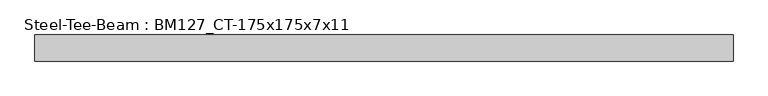
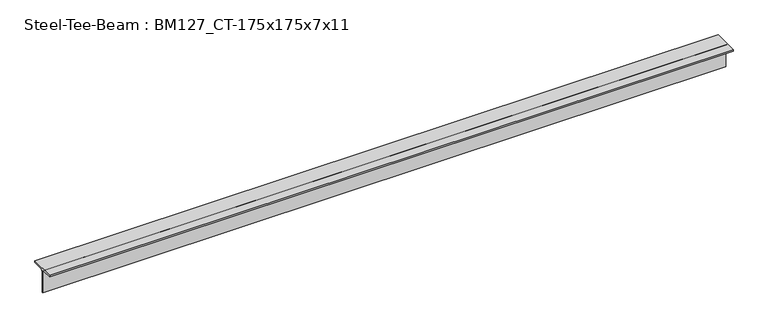
"""IFC4 building model written with IfcOpenShell, lengths in millimetres: beam geometry, Steel-Tee-Beam : BM127_CT-175x175x7x11."""

from ifc_helpers import new_model, si_unit, point, frame, frame_2d, origin, place, context, project, spatial, polyline, circle_curve, trimmed, segment, composite_curve, outline, extrude, source, transform, mapped, element, save


def steel_tee_beam_bm127_ct_175x175x7x11_ea611a39(model_context):
    return source(origin(), model_context, "Body", "SweptSolid", [
        extrude(outline(composite_curve([segment(polyline([(87.5, 87.5), (87.5, 76.5), (17.5, 76.5)]), True, "CONTINUOUS"), segment(trimmed(circle_curve(frame_2d((17.5, 62.5)), 14.0), [point((17.5, 76.5))], [point((3.5, 62.5))], True, "CARTESIAN"), True, "CONTINUOUS"), segment(polyline([(3.5, 62.5), (3.5, -87.5), (-3.5, -87.5), (-3.5, 62.5)]), True, "CONTINUOUS"), segment(trimmed(circle_curve(frame_2d((-17.5, 62.5)), 14.0), [point((-3.5, 62.5))], [point((-17.5, 76.5))], True, "CARTESIAN"), True, "CONTINUOUS"), segment(polyline([(-17.5, 76.5), (-87.5, 76.5), (-87.5, 87.5), (87.5, 87.5)]), True, "CONTINUOUS")], self_intersect=False)), frame((-2302.448777, 0.0, 0.0), z_axis=(1.0, 0.0, 0.0), x_axis=(0.0, 1.0, 0.0)), (0.0, 0.0, 1.0), 4667.7067484),
    ])


if __name__ == "__main__":
    model = new_model("IFC4")
    model_context = context("Model", 3, world=origin())
    ifc_project = project(units=[si_unit("LENGTHUNIT", "METRE", prefix="MILLI")], contexts=[model_context])
    site = spatial("IfcSite", under=ifc_project)
    building = spatial("IfcBuilding", under=site)
    placement = place(None, origin())
    steel_tee_beam_bm127_ct_175x175x7x11_shape = steel_tee_beam_bm127_ct_175x175x7x11_ea611a39(model_context)
    element("IfcBeam", 1, ObjectType="Steel-Tee-Beam : BM127_CT-175x175x7x11", at=placement, inside=building, context=model_context, shape_type="MappedRepresentation", body=[
        mapped(steel_tee_beam_bm127_ct_175x175x7x11_shape, transform((0.0, 0.0, 0.0), x_axis=(1.0, 0.0, 0.0), y_axis=(0.0, 1.0, 0.0), z_axis=(0.0, 0.0, 1.0))),
    ])
    save(model, "model.ifc")

# Revit data of these elements
# Type "Steel-Tee-Beam : BM127_CT-175x175x7x11"
#   Surface Area = 0.00 m²/m
#   Section Area = 31.57 cm²
#   Mass per Unit Length = 24.80 kg/m
#   Length [instance default] = 1524 mm
#   bf = 175 mm
#   d = 175 mm
#   k = 25 mm
#   kr = 14 mm
#   tf = 11 mm
#   tw = 7 mm
#   hec_material4 [instance default] = none
#   hec_material3 [instance default] = none
#   hec_material2 [instance default] = none
#   hec_material1 [instance default] = none
#   Structural Material [instance default] = Steel, 45-345
#   Assembly Code = ""
# Element 1 (IfcBeam, "Steel-Tee-Beam : BM127_CT-175x175x7x11")
#   hec_material3 = F01AC000-00002_Building/Shelter Fire Proofing Work_Intumescent Coating Type_1 hr. rating (UL 1709))
#   hec_material2 = S01AA010-00002_Main Steel Structure Fabrication Work_Shelter/Building_Steel Painting/Coating_for Fireproofed Steel Surface, Surface Preparation & Primer Coat
#   hec_material1 = S03AA029-00001_Main Steel Structure Erection Work_Shelter/Building_Light Steel
#   Structural Material = S01AA003-00001_Main Steel Structure Fabrication Work_Shelter/Building_Light Steel - Standard
#   Materials on its faces: "S01AA003-00001_Main Steel Structure Fabrication Work_Shelter/Building_Light Steel - Standard"
# Materials
#   "Steel, 45-345": class "Metal", colour RGB 189 187 185, transparency 0, Description = "Steel 345 MPa", Cost = 0
#   "S01AA003-00001_Main Steel Structure Fabrication Work_Shelter/Building_Light Steel - Standard": class "Metal", colour RGB 120 120 120, transparency 0, Comments = "(30KG/M>Weight)", Description = "Structural steel 50ksi", W00) Work Master Code = "S01AA003-00001", W01) Work Master_Lv1 = "Main Steel Structure Fabrication Work", W02) Work Master_Lv2 = "Shelter/Building", W03) Work Master_Spec.1 = "Light Steel - Standard (30KG/M>Weight)", Cost = 0
#   "F01AC000-00002_Building/Shelter Fire Proofing Work_Intumescent Coating Type_1 hr. rating (UL 1709))": class "Metal", colour RGB 255 128 128, transparency 0, Description = "Paint finished steel", W00) Work Master Code = "F01AC000-00002", W01) Work Master_Lv1 = "Building/Shelter Fire Proofing Work", W02) Work Master_Lv2 = "Intumescent Coating Type", W03) Work Master_Spec.1 = "1 hr. rating (UL 1709)", Cost = 0
#   "S01AA010-00002_Main Steel Structure Fabrication Work_Shelter/Building_Steel Painting/Coating_for Fireproofed Steel Surface, Surface Preparation & Primer Coat": class "Metal", colour RGB 120 120 120, transparency 0, Description = "Paint finished steel", W00) Work Master Code = "SS01AA010-00002", W01) Work Master_Lv1 = "Main Steel Structure Fabrication Work", W02) Work Master_Lv2 = "Shelter/Building", W03) Work Master_Spec.1 = "Steel Painting/Coating", W04) Work Master_Spec.2 = "for Fireproofed Steel Surface, Surface Preparation & Primer Coat", Cost = 0
#   "S03AA029-00001_Main Steel Structure Erection Work_Shelter/Building_Light Steel": class "Metal", colour RGB 120 120 120, transparency 0, Comments = "(30KG/M>Weight)", Description = "Structural steel 50ksi", W00) Work Master Code = "S03AA029-00001", W01) Work Master_Lv1 = "Main Steel Structure Erection Work", W02) Work Master_Lv2 = "Shelter/Building", W03) Work Master_Spec.1 = "Light Steel (30KG/M>Weight)", Cost = 0
